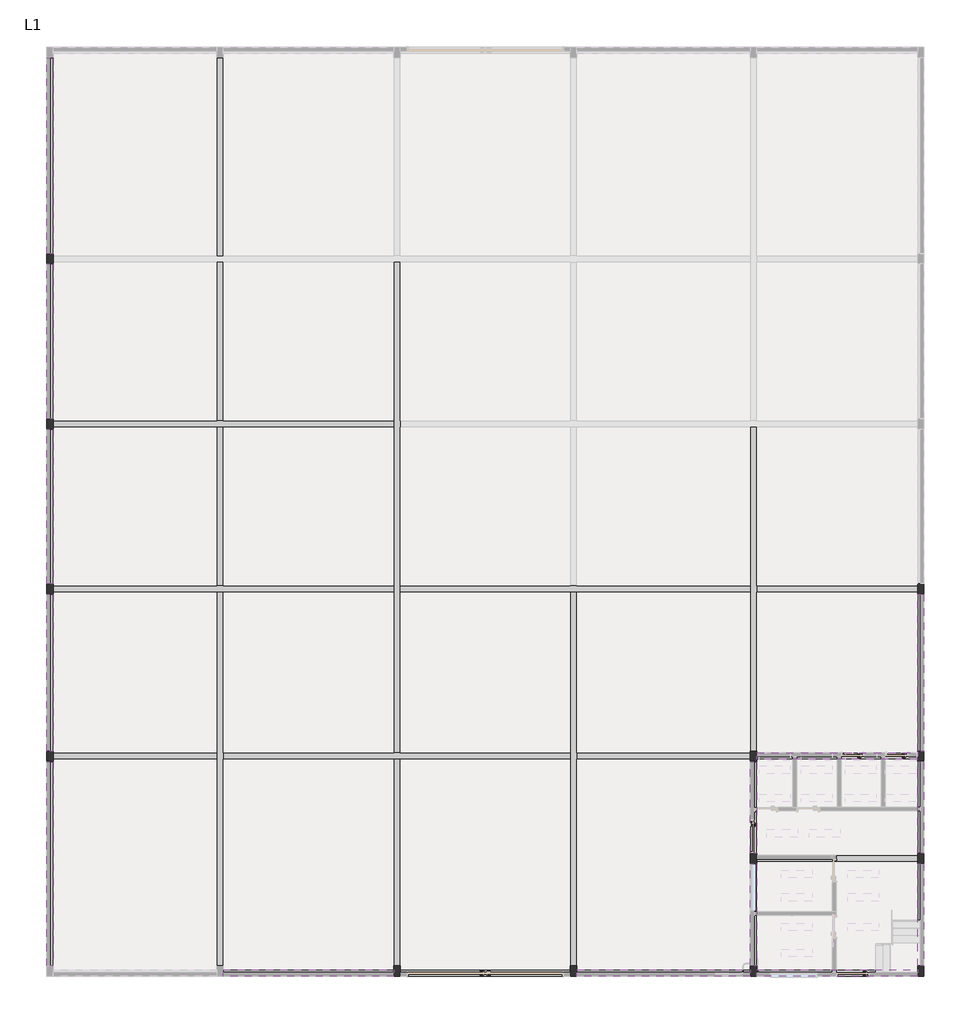
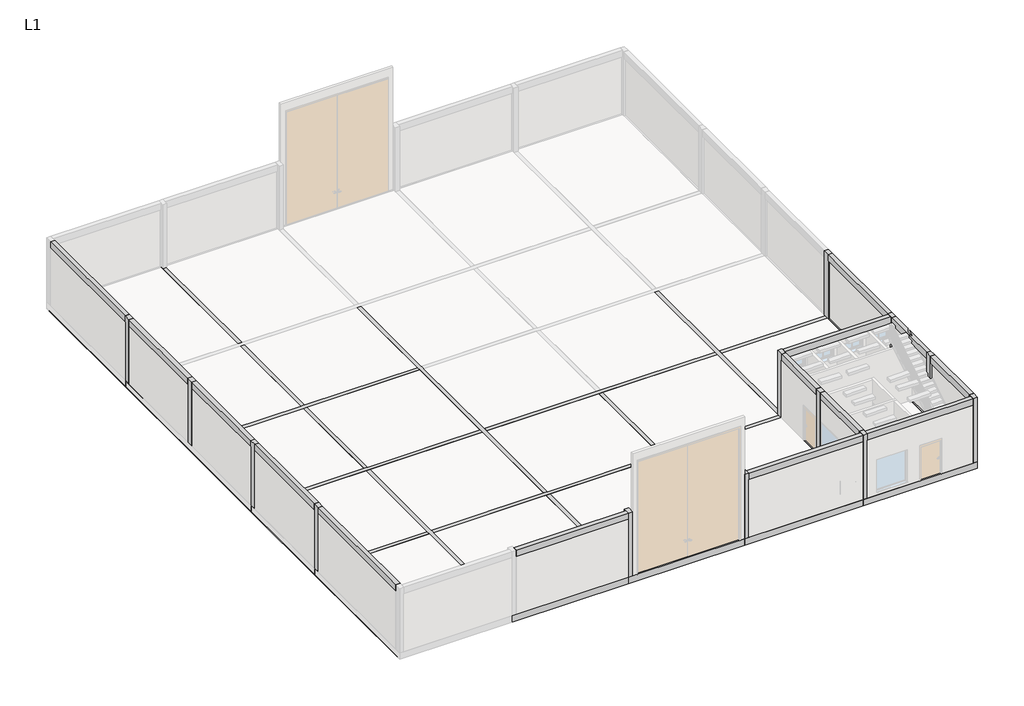
# One storey, part 2 of 4: 45 beams, 13 columns.
"""IFC4 building model written with IfcOpenShell, lengths in millimetres."""

from ifc_helpers import new_model, si_unit, frame, origin, place, context, project, spatial, polyline, outline, extrude, faceted_brep, element, save

model = new_model("IFC4")

# Units and contexts
model_context = context("Model", 3, world=origin())
ifc_project = project(units=[si_unit("LENGTHUNIT", "METRE", prefix="MILLI")], contexts=[model_context])

# Site, building, storey
site = spatial("IfcSite", under=ifc_project)
building = spatial("IfcBuilding", under=site)
storey = spatial("IfcBuildingStorey", under=building, Name="L1", Elevation=0.0)

# Beams
placement = place(None, origin())
element("IfcBeam", 1, ObjectType="M_Hormigón-Viga rectangular : 250 x 400mm", at=placement, inside=storey, context=model_context, shape_type="Brep", body=[
    faceted_brep([(17000.0, -3125.0, 0.0), (17000.0, -2875.0, 0.0), (16750.0, -2875.0, 0.0), (10525.0, -2875.0, 0.0), (10525.0, -3125.0, 0.0), (16750.0, -3125.0, 0.0), (17000.0, -2875.0, -400.0), (16750.0, -2875.0, -400.0), (10525.0, -2875.0, -400.0), (10525.0, -2875.0, -350.0), (17000.0, -3125.0, -400.0), (16750.0, -3125.0, -400.0), (10525.0, -3125.0, -400.0), (10525.0, -3125.0, -350.0)], [[[0, 1, 2, 3, 4, 5]], [[1, 6, 7, 8, 9, 3, 2]], [[6, 10, 11, 12, 8, 7]], [[10, 0, 5, 4, 13, 12, 11]], [[1, 0, 10, 6]], [[4, 3, 9, 8, 12, 13]]]),
])
element("IfcBeam", 2, ObjectType="M_Hormigón-Viga rectangular : 250 x 400mm", at=placement, inside=storey, context=model_context, shape_type="Brep", body=[
    faceted_brep([(10275.0, -9345.0, 0.0), (10275.0, -9595.0, 0.0), (10525.0, -9595.0, 0.0), (16750.0, -9595.0, 0.0), (17000.0, -9595.0, 0.0), (17000.0, -9345.0, 0.0), (16750.0, -9345.0, 0.0), (10525.0, -9345.0, 0.0), (10275.0, -9345.0, -400.0), (17000.0, -9345.0, -400.0), (16750.0, -9345.0, -400.0), (10525.0, -9345.0, -400.0), (10275.0, -9595.0, -400.0), (17000.0, -9595.0, -400.0), (16750.0, -9595.0, -400.0), (10525.0, -9595.0, -400.0)], [[[0, 1, 2, 3, 4, 5, 6, 7]], [[8, 0, 7, 6, 5, 9, 10, 11]], [[12, 8, 11, 10, 9, 13, 14, 15]], [[1, 12, 15, 14, 13, 4, 3, 2]], [[1, 0, 8, 12]], [[5, 4, 13, 9]]]),
])
element("IfcBeam", 3, ObjectType="M_Hormigón-Viga rectangular : 250 x 400mm", at=placement, inside=storey, context=model_context, shape_type="Brep", body=[
    faceted_brep([(10275.0, -9595.0, 0.0), (10275.0, -9345.0, 0.0), (3550.0, -9345.0, 0.0), (3550.0, -9595.0, 0.0), (10275.0, -9345.0, -350.0), (10275.0, -9345.0, -400.0), (3550.0, -9345.0, -400.0), (3550.0, -9345.0, -350.0), (10275.0, -9595.0, -400.0), (3550.0, -9595.0, -400.0), (10275.0, -9595.0, -350.0), (3550.0, -9595.0, -350.0)], [[[0, 1, 2, 3]], [[1, 4, 5, 6, 7, 2]], [[5, 8, 9, 6]], [[8, 10, 0, 3, 11, 9]], [[1, 0, 10, 8, 5, 4]], [[3, 2, 7, 6, 9, 11]]]),
])
element("IfcBeam", 4, ObjectType="M_Hormigón-Viga rectangular : 250 x 400mm", at=placement, inside=storey, context=model_context, shape_type="Brep", body=[
    faceted_brep([(10275.0, -17750.0, 0.0), (10275.0, -18000.0, 0.0), (17000.0, -18000.0, 0.0), (17000.0, -17750.0, 0.0), (16750.0, -17750.0, 0.0), (10525.0, -17750.0, 0.0), (10275.0, -17750.0, -400.0), (17000.0, -17750.0, -400.0), (16750.0, -17750.0, -400.0), (10525.0, -17750.0, -400.0), (10275.0, -18000.0, -400.0), (17000.0, -18000.0, -400.0)], [[[0, 1, 2, 3, 4, 5]], [[6, 0, 5, 4, 3, 7, 8, 9]], [[10, 6, 9, 8, 7, 11]], [[1, 10, 11, 2]], [[1, 0, 6, 10]], [[3, 2, 11, 7]]]),
])
element("IfcBeam", 5, ObjectType="M_Hormigón-Viga rectangular : 250 x 400mm", at=placement, inside=storey, context=model_context, shape_type="Brep", body=[
    faceted_brep([(3300.0, -17750.0, 0.0), (3300.0, -18000.0, 0.0), (10275.0, -18000.0, 0.0), (10275.0, -17750.0, 0.0), (3550.0, -17750.0, 0.0), (3300.0, -17750.0, -400.0), (10275.0, -17750.0, -350.0), (10275.0, -17750.0, -400.0), (3550.0, -17750.0, -400.0), (3300.0, -18000.0, -400.0), (10275.0, -18000.0, -400.0)], [[[0, 1, 2, 3, 4]], [[5, 0, 4, 3, 6, 7, 8]], [[9, 5, 8, 7, 10]], [[1, 9, 10, 2]], [[1, 0, 5, 9]], [[3, 2, 10, 7, 6]]]),
])
element("IfcBeam", 6, ObjectType="M_Hormigón-Viga rectangular : 250 x 400mm", at=placement, inside=storey, context=model_context, shape_type="Brep", body=[
    faceted_brep([(-3550.0, -17750.0, 0.0), (-3550.0, -18000.0, 0.0), (3300.0, -18000.0, 0.0), (3300.0, -17750.0, 0.0), (-3300.0, -17750.0, 0.0), (-3550.0, -17750.0, -400.0), (3300.0, -17750.0, -350.0), (3300.0, -17750.0, -400.0), (-3300.0, -17750.0, -400.0), (-3550.0, -18000.0, -400.0), (3300.0, -18000.0, -400.0)], [[[0, 1, 2, 3, 4]], [[5, 0, 4, 3, 6, 7, 8]], [[9, 5, 8, 7, 10]], [[1, 9, 10, 2]], [[1, 0, 5, 9]], [[3, 2, 10, 7, 6]]]),
])
element("IfcBeam", 7, ObjectType="M_Hormigón-Viga rectangular : 250 x 400mm", at=placement, inside=storey, context=model_context, shape_type="Brep", body=[
    faceted_brep([(-10400.0, -17750.0, 0.0), (-10400.0, -18000.0, 0.0), (-3550.0, -18000.0, 0.0), (-3550.0, -17750.0, 0.0), (-10150.0, -17750.0, 0.0), (-10400.0, -17750.0, -400.0), (-3550.0, -17750.0, -350.0), (-3550.0, -17750.0, -400.0), (-10150.0, -17750.0, -400.0), (-10400.0, -18000.0, -400.0), (-3550.0, -18000.0, -400.0)], [[[0, 1, 2, 3, 4]], [[5, 0, 4, 3, 6, 7, 8]], [[9, 5, 8, 7, 10]], [[1, 9, 10, 2]], [[3, 2, 10, 7, 6]], [[1, 0, 5, 9]]]),
])
element("IfcBeam", 8, ObjectType="M_Hormigón-Viga rectangular : 250 x 400mm", at=placement, inside=storey, context=model_context, shape_type="Brep", body=[
    faceted_brep([(-16750.0, -9345.0, 0.0), (-17000.0, -9345.0, 0.0), (-17000.0, -9685.0, 0.0), (-17000.0, -17600.0, 0.0), (-17000.0, -17750.0, 0.0), (-16750.0, -17750.0, 0.0), (-16750.0, -17600.0, 0.0), (-16750.0, -9685.0, 0.0), (-16750.0, -9595.0, 0.0), (-16750.0, -9345.0, -400.0), (-16750.0, -17750.0, -350.0), (-16750.0, -17750.0, -400.0), (-16750.0, -9595.0, -400.0), (-17000.0, -9345.0, -400.0), (-17000.0, -17750.0, -400.0)], [[[0, 1, 2, 3, 4, 5, 6, 7, 8]], [[9, 0, 8, 7, 6, 5, 10, 11, 12]], [[13, 9, 12, 11, 14]], [[1, 13, 14, 4, 3, 2]], [[1, 0, 9, 13]], [[5, 4, 14, 11, 10]]]),
])
element("IfcBeam", 9, ObjectType="M_Hormigón-Viga rectangular : 250 x 400mm", at=placement, inside=storey, context=model_context, shape_type="Brep", body=[
    faceted_brep([(-16750.0, -2875.0, 0.0), (-17000.0, -2875.0, 0.0), (-17000.0, -3200.0, 0.0), (-17000.0, -9285.0, 0.0), (-17000.0, -9345.0, 0.0), (-16750.0, -9345.0, 0.0), (-16750.0, -9285.0, 0.0), (-16750.0, -3200.0, 0.0), (-16750.0, -3125.0, 0.0), (-16750.0, -2875.0, -400.0), (-16750.0, -9345.0, -350.0), (-16750.0, -9345.0, -400.0), (-16750.0, -3125.0, -400.0), (-17000.0, -2875.0, -400.0), (-17000.0, -9345.0, -400.0)], [[[0, 1, 2, 3, 4, 5, 6, 7, 8]], [[9, 0, 8, 7, 6, 5, 10, 11, 12]], [[13, 9, 12, 11, 14]], [[1, 13, 14, 4, 3, 2]], [[1, 0, 9, 13]], [[5, 4, 14, 11, 10]]]),
])
element("IfcBeam", 10, ObjectType="M_Hormigón-Viga rectangular : 250 x 400mm", at=placement, inside=storey, context=model_context, shape_type="Brep", body=[
    faceted_brep([(-16750.0, 3525.0, 0.0), (-17000.0, 3525.0, 0.0), (-17000.0, 3200.0, 0.0), (-17000.0, -2800.0, 0.0), (-17000.0, -2875.0, 0.0), (-16750.0, -2875.0, 0.0), (-16750.0, -2800.0, 0.0), (-16750.0, 3200.0, 0.0), (-16750.0, 3275.0, 0.0), (-16750.0, 3525.0, -400.0), (-16750.0, -2875.0, -350.0), (-16750.0, -2875.0, -400.0), (-16750.0, 3275.0, -400.0), (-17000.0, 3525.0, -400.0), (-17000.0, -2875.0, -400.0)], [[[0, 1, 2, 3, 4, 5, 6, 7, 8]], [[9, 0, 8, 7, 6, 5, 10, 11, 12]], [[13, 9, 12, 11, 14]], [[1, 13, 14, 4, 3, 2]], [[1, 0, 9, 13]], [[5, 4, 14, 11, 10]]]),
])
element("IfcBeam", 11, ObjectType="M_Hormigón-Viga rectangular : 250 x 400mm", at=placement, inside=storey, context=model_context, shape_type="Brep", body=[
    faceted_brep([(-16750.0, 9925.0, 0.0), (-17000.0, 9925.0, 0.0), (-17000.0, 9600.0, 0.0), (-17000.0, 3600.0, 0.0), (-17000.0, 3525.0, 0.0), (-16750.0, 3525.0, 0.0), (-16750.0, 3600.0, 0.0), (-16750.0, 9600.0, 0.0), (-16750.0, 9675.0, 0.0), (-16750.0, 9925.0, -400.0), (-16750.0, 3525.0, -350.0), (-16750.0, 3525.0, -400.0), (-16750.0, 9675.0, -400.0), (-17000.0, 9925.0, -400.0), (-17000.0, 3525.0, -400.0)], [[[0, 1, 2, 3, 4, 5, 6, 7, 8]], [[9, 0, 8, 7, 6, 5, 10, 11, 12]], [[13, 9, 12, 11, 14]], [[1, 13, 14, 4, 3, 2]], [[1, 0, 9, 13]], [[5, 4, 14, 11, 10]]]),
])
element("IfcBeam", 12, ObjectType="M_Hormigón-Viga rectangular : 250 x 400mm", at=placement, inside=storey, context=model_context, shape_type="Brep", body=[
    faceted_brep([(-16750.0, 17750.0, 0.0), (-17000.0, 17750.0, 0.0), (-17000.0, 17600.0, 0.0), (-17000.0, 10000.0, 0.0), (-17000.0, 9925.0, 0.0), (-16750.0, 9925.0, 0.0), (-16750.0, 10000.0, 0.0), (-16750.0, 17600.0, 0.0), (-16750.0, 17750.0, -400.0), (-16750.0, 17750.0, -350.0), (-16750.0, 9925.0, -350.0), (-16750.0, 9925.0, -400.0), (-17000.0, 17750.0, -400.0), (-17000.0, 9925.0, -400.0)], [[[0, 1, 2, 3, 4, 5, 6, 7]], [[8, 9, 0, 7, 6, 5, 10, 11]], [[12, 8, 11, 13]], [[1, 12, 13, 4, 3, 2]], [[1, 0, 9, 8, 12]], [[5, 4, 13, 11, 10]]]),
])
element("IfcBeam", 13, ObjectType="M_Hormigón-Viga rectangular : 250 x 400mm", at=placement, inside=storey, context=model_context, shape_type="Brep", body=[
    faceted_brep([(-3550.0, -17750.0, 0.0), (-3300.0, -17750.0, 0.0), (-3300.0, -9595.0, 0.0), (-3550.0, -9595.0, 0.0), (-3300.0, -17750.0, -350.0), (-3300.0, -17750.0, -400.0), (-3300.0, -9595.0, -400.0), (-3300.0, -9595.0, -350.0), (-3550.0, -17750.0, -400.0), (-3550.0, -9595.0, -400.0), (-3550.0, -17750.0, -350.0), (-3550.0, -9595.0, -350.0)], [[[0, 1, 2, 3]], [[1, 4, 5, 6, 7, 2]], [[5, 8, 9, 6]], [[8, 10, 0, 3, 11, 9]], [[1, 0, 10, 8, 5, 4]], [[3, 2, 7, 6, 9, 11]]]),
])
element("IfcBeam", 14, ObjectType="M_Hormigón-Viga rectangular : 250 x 400mm", at=placement, inside=storey, context=model_context, shape_type="Brep", body=[
    faceted_brep([(3300.0, -17750.0, 0.0), (3550.0, -17750.0, 0.0), (3550.0, -9595.0, 0.0), (3550.0, -9345.0, 0.0), (3550.0, -3125.0, 0.0), (3300.0, -3125.0, 0.0), (3300.0, -9345.0, 0.0), (3300.0, -9595.0, 0.0), (3550.0, -17750.0, -350.0), (3550.0, -17750.0, -400.0), (3550.0, -9595.0, -400.0), (3550.0, -9345.0, -400.0), (3550.0, -3125.0, -400.0), (3550.0, -3125.0, -350.0), (3300.0, -17750.0, -400.0), (3300.0, -9595.0, -400.0), (3300.0, -9345.0, -400.0), (3300.0, -3125.0, -400.0), (3300.0, -17750.0, -350.0), (3300.0, -3125.0, -350.0)], [[[0, 1, 2, 3, 4, 5, 6, 7]], [[1, 8, 9, 10, 11, 12, 13, 4, 3, 2]], [[9, 14, 15, 16, 17, 12, 11, 10]], [[14, 18, 0, 7, 6, 5, 19, 17, 16, 15]], [[1, 0, 18, 14, 9, 8]], [[5, 4, 13, 12, 17, 19]]]),
])
element("IfcBeam", 15, ObjectType="M_Hormigón-Viga rectangular : 250 x 400mm", at=placement, inside=storey, context=model_context, shape_type="Brep", body=[
    faceted_brep([(10525.0, -13315.5675387, 0.0), (10275.0, -13315.5675387, 0.0), (10275.0, -17750.0, 0.0), (10525.0, -17750.0, 0.0), (10525.0, -13565.5675387, 0.0), (10525.0, -13315.5675387, -400.0), (10525.0, -17750.0, -350.0), (10525.0, -17750.0, -400.0), (10275.0, -13315.5675387, -400.0), (10275.0, -17750.0, -400.0), (10275.0, -17750.0, -350.0)], [[[0, 1, 2, 3, 4]], [[5, 0, 4, 3, 6, 7]], [[8, 5, 7, 9]], [[1, 8, 9, 10, 2]], [[3, 2, 10, 9, 7, 6]], [[1, 0, 5, 8]]]),
])
element("IfcBeam", 16, ObjectType="M_Hormigón-Viga rectangular : 250 x 400mm", at=placement, inside=storey, context=model_context, shape_type="Brep", body=[
    faceted_brep([(10525.0, -9595.0, 0.0), (10275.0, -9595.0, 0.0), (10275.0, -13315.5675387, 0.0), (10525.0, -13315.5675387, 0.0), (10525.0, -9595.0, -400.0), (10525.0, -9595.0, -350.0), (10525.0, -13315.5675387, -350.0), (10525.0, -13315.5675387, -400.0), (10275.0, -9595.0, -400.0), (10275.0, -13315.5675387, -400.0), (10275.0, -9595.0, -350.0)], [[[0, 1, 2, 3]], [[4, 5, 0, 3, 6, 7]], [[8, 4, 7, 9]], [[1, 10, 8, 9, 2]], [[1, 0, 5, 4, 8, 10]], [[3, 2, 9, 7, 6]]]),
])
element("IfcBeam", 17, ObjectType="M_Hormigón-Viga rectangular : 250 x 400mm", at=placement, inside=storey, context=model_context, shape_type="Brep", body=[
    faceted_brep([(10275.0, -9345.0, 0.0), (10525.0, -9345.0, 0.0), (10525.0, -3125.0, 0.0), (10525.0, -2875.0, 0.0), (10525.0, 3275.0, 0.0), (10275.0, 3275.0, 0.0), (10275.0, -2875.0, 0.0), (10275.0, -3125.0, 0.0), (10525.0, -9345.0, -350.0), (10525.0, -9345.0, -400.0), (10525.0, -3125.0, -400.0), (10525.0, -2875.0, -400.0), (10525.0, 3275.0, -400.0), (10525.0, 3275.0, -350.0), (10275.0, -9345.0, -400.0), (10275.0, -3125.0, -400.0), (10275.0, -2875.0, -400.0), (10275.0, 3275.0, -400.0), (10275.0, -9345.0, -350.0), (10275.0, 3275.0, -350.0)], [[[0, 1, 2, 3, 4, 5, 6, 7]], [[1, 8, 9, 10, 11, 12, 13, 4, 3, 2]], [[9, 14, 15, 16, 17, 12, 11, 10]], [[14, 18, 0, 7, 6, 5, 19, 17, 16, 15]], [[1, 0, 18, 14, 9, 8]], [[5, 4, 13, 12, 17, 19]]]),
])
element("IfcBeam", 18, ObjectType="M_Hormigón-Viga rectangular : 250 x 400mm", at=placement, inside=storey, context=model_context, shape_type="Brep", body=[
    faceted_brep([(17000.0, -13315.5675387, 0.0), (16750.0, -13315.5675387, 0.0), (16750.0, -13565.5675387, 0.0), (16750.0, -13640.5675387, 0.0), (16750.0, -17600.0, 0.0), (16750.0, -17750.0, 0.0), (17000.0, -17750.0, 0.0), (17000.0, -17600.0, 0.0), (17000.0, -13640.5675387, 0.0), (17000.0, -13315.5675387, -400.0), (17000.0, -17750.0, -400.0), (16750.0, -13315.5675387, -400.0), (16750.0, -17750.0, -400.0), (16750.0, -13565.5675387, -400.0), (16750.0, -17750.0, -350.0)], [[[0, 1, 2, 3, 4, 5, 6, 7, 8]], [[9, 0, 8, 7, 6, 10]], [[11, 9, 10, 12, 13]], [[1, 11, 13, 12, 14, 5, 4, 3, 2]], [[6, 5, 14, 12, 10]], [[1, 0, 9, 11]]]),
])
element("IfcBeam", 19, ObjectType="M_Hormigón-Viga rectangular : 250 x 400mm", at=placement, inside=storey, context=model_context, shape_type="Brep", body=[
    faceted_brep([(17000.0, -9595.0, 0.0), (16750.0, -9595.0, 0.0), (16750.0, -9685.0, 0.0), (16750.0, -13240.5675387, 0.0), (16750.0, -13315.5675387, 0.0), (17000.0, -13315.5675387, 0.0), (17000.0, -13240.5675387, 0.0), (17000.0, -9685.0, 0.0), (17000.0, -9595.0, -400.0), (17000.0, -13315.5675387, -400.0), (16750.0, -9595.0, -400.0), (16750.0, -13315.5675387, -400.0), (16750.0, -9595.0, -350.0), (16750.0, -13315.5675387, -350.0)], [[[0, 1, 2, 3, 4, 5, 6, 7]], [[8, 0, 7, 6, 5, 9]], [[10, 8, 9, 11]], [[1, 12, 10, 11, 13, 4, 3, 2]], [[1, 0, 8, 10, 12]], [[5, 4, 13, 11, 9]]]),
])
element("IfcBeam", 20, ObjectType="M_Hormigón-Viga rectangular : 250 x 400mm", at=placement, inside=storey, context=model_context, shape_type="Brep", body=[
    faceted_brep([(17000.0, -3125.0, 0.0), (16750.0, -3125.0, 0.0), (16750.0, -3200.0, 0.0), (16750.0, -9285.0, 0.0), (16750.0, -9345.0, 0.0), (17000.0, -9345.0, 0.0), (17000.0, -9285.0, 0.0), (17000.0, -3200.0, 0.0), (17000.0, -3125.0, -400.0), (17000.0, -9345.0, -400.0), (16750.0, -3125.0, -400.0), (16750.0, -9345.0, -400.0), (16750.0, -3125.0, -350.0), (16750.0, -9345.0, -350.0)], [[[0, 1, 2, 3, 4, 5, 6, 7]], [[8, 0, 7, 6, 5, 9]], [[10, 8, 9, 11]], [[1, 12, 10, 11, 13, 4, 3, 2]], [[1, 0, 8, 10, 12]], [[5, 4, 13, 11, 9]]]),
])
element("IfcBeam", 21, ObjectType="M_Hormigón-Viga rectangular : 250 x 400mm", at=placement, inside=storey, context=model_context, shape_type="Brep", body=[
    faceted_brep([(-10400.0, -17750.0, 0.0), (-10150.0, -17750.0, 0.0), (-10150.0, -9595.0, 0.0), (-10150.0, -9345.0, 0.0), (-10150.0, -3125.0, 0.0), (-10400.0, -3125.0, 0.0), (-10400.0, -9345.0, 0.0), (-10400.0, -9595.0, 0.0), (-10150.0, -17750.0, -350.0), (-10150.0, -17750.0, -400.0), (-10150.0, -9595.0, -400.0), (-10150.0, -9345.0, -400.0), (-10150.0, -3125.0, -400.0), (-10150.0, -3125.0, -350.0), (-10400.0, -17750.0, -400.0), (-10400.0, -9595.0, -400.0), (-10400.0, -9345.0, -400.0), (-10400.0, -3125.0, -400.0), (-10400.0, -17750.0, -350.0), (-10400.0, -3125.0, -350.0)], [[[0, 1, 2, 3, 4, 5, 6, 7]], [[1, 8, 9, 10, 11, 12, 13, 4, 3, 2]], [[9, 14, 15, 16, 17, 12, 11, 10]], [[14, 18, 0, 7, 6, 5, 19, 17, 16, 15]], [[1, 0, 18, 14, 9, 8]], [[5, 4, 13, 12, 17, 19]]]),
])
element("IfcBeam", 22, ObjectType="M_Hormigón-Viga rectangular : 250 x 400mm", at=placement, inside=storey, context=model_context, shape_type="Brep", body=[
    faceted_brep([(-16750.0, 3525.0, 0.0), (-16750.0, 3275.0, 0.0), (-10400.0, 3275.0, 0.0), (-10150.0, 3275.0, 0.0), (-3550.0, 3275.0, 0.0), (-3550.0, 3525.0, 0.0), (-10150.0, 3525.0, 0.0), (-10400.0, 3525.0, 0.0), (-16750.0, 3525.0, -400.0), (-16750.0, 3525.0, -350.0), (-3550.0, 3525.0, -350.0), (-3550.0, 3525.0, -400.0), (-10150.0, 3525.0, -400.0), (-10400.0, 3525.0, -400.0), (-16750.0, 3275.0, -400.0), (-3550.0, 3275.0, -400.0), (-10150.0, 3275.0, -400.0), (-10400.0, 3275.0, -400.0), (-16750.0, 3275.0, -350.0), (-3550.0, 3275.0, -350.0)], [[[0, 1, 2, 3, 4, 5, 6, 7]], [[8, 9, 0, 7, 6, 5, 10, 11, 12, 13]], [[14, 8, 13, 12, 11, 15, 16, 17]], [[1, 18, 14, 17, 16, 15, 19, 4, 3, 2]], [[1, 0, 9, 8, 14, 18]], [[5, 4, 19, 15, 11, 10]]]),
])
element("IfcBeam", 23, ObjectType="M_Hormigón-Viga rectangular : 250 x 400mm", at=placement, inside=storey, context=model_context, shape_type="Brep", body=[
    faceted_brep([(-16750.0, -2875.0, 0.0), (-16750.0, -3125.0, 0.0), (-10400.0, -3125.0, 0.0), (-10150.0, -3125.0, 0.0), (-3550.0, -3125.0, 0.0), (-3550.0, -2875.0, 0.0), (-10150.0, -2875.0, 0.0), (-10400.0, -2875.0, 0.0), (-16750.0, -2875.0, -400.0), (-16750.0, -2875.0, -350.0), (-3550.0, -2875.0, -350.0), (-3550.0, -2875.0, -400.0), (-10150.0, -2875.0, -400.0), (-10400.0, -2875.0, -400.0), (-16750.0, -3125.0, -400.0), (-3550.0, -3125.0, -400.0), (-10150.0, -3125.0, -400.0), (-10400.0, -3125.0, -400.0), (-16750.0, -3125.0, -350.0), (-3550.0, -3125.0, -350.0)], [[[0, 1, 2, 3, 4, 5, 6, 7]], [[8, 9, 0, 7, 6, 5, 10, 11, 12, 13]], [[14, 8, 13, 12, 11, 15, 16, 17]], [[1, 18, 14, 17, 16, 15, 19, 4, 3, 2]], [[1, 0, 9, 8, 14, 18]], [[5, 4, 19, 15, 11, 10]]]),
])
element("IfcBeam", 24, ObjectType="M_Hormigón-Viga rectangular : 250 x 400mm", at=placement, inside=storey, context=model_context, shape_type="Brep", body=[
    faceted_brep([(-3300.0, -2875.0, 0.0), (-3300.0, -3125.0, 0.0), (3300.0, -3125.0, 0.0), (3550.0, -3125.0, 0.0), (10275.0, -3125.0, 0.0), (10275.0, -2875.0, 0.0), (3550.0, -2875.0, 0.0), (3300.0, -2875.0, 0.0), (-3300.0, -2875.0, -400.0), (-3300.0, -2875.0, -350.0), (10275.0, -2875.0, -350.0), (10275.0, -2875.0, -400.0), (3550.0, -2875.0, -400.0), (3300.0, -2875.0, -400.0), (-3300.0, -3125.0, -400.0), (10275.0, -3125.0, -400.0), (3550.0, -3125.0, -400.0), (3300.0, -3125.0, -400.0), (-3300.0, -3125.0, -350.0), (10275.0, -3125.0, -350.0)], [[[0, 1, 2, 3, 4, 5, 6, 7]], [[8, 9, 0, 7, 6, 5, 10, 11, 12, 13]], [[14, 8, 13, 12, 11, 15, 16, 17]], [[1, 18, 14, 17, 16, 15, 19, 4, 3, 2]], [[1, 0, 9, 8, 14, 18]], [[5, 4, 19, 15, 11, 10]]]),
])
element("IfcBeam", 25, ObjectType="M_Hormigón-Viga rectangular : 250 x 400mm", at=placement, inside=storey, context=model_context, shape_type="Brep", body=[
    faceted_brep([(-3300.0, 9675.0, 0.0), (-3550.0, 9675.0, 0.0), (-3550.0, 3525.0, 0.0), (-3550.0, 3275.0, 0.0), (-3550.0, -2875.0, 0.0), (-3550.0, -3125.0, 0.0), (-3550.0, -9345.0, 0.0), (-3300.0, -9345.0, 0.0), (-3300.0, -3125.0, 0.0), (-3300.0, -2875.0, 0.0), (-3300.0, 3275.0, 0.0), (-3300.0, 3525.0, 0.0), (-3300.0, 9675.0, -400.0), (-3300.0, 9675.0, -350.0), (-3300.0, -9345.0, -350.0), (-3300.0, -9345.0, -400.0), (-3300.0, -3125.0, -400.0), (-3300.0, -2875.0, -400.0), (-3300.0, 3275.0, -400.0), (-3300.0, 3525.0, -400.0), (-3550.0, 9675.0, -400.0), (-3550.0, -9345.0, -400.0), (-3550.0, -3125.0, -400.0), (-3550.0, -2875.0, -400.0), (-3550.0, 3275.0, -400.0), (-3550.0, 3525.0, -400.0), (-3550.0, 9675.0, -350.0), (-3550.0, -9345.0, -350.0)], [[[0, 1, 2, 3, 4, 5, 6, 7, 8, 9, 10, 11]], [[12, 13, 0, 11, 10, 9, 8, 7, 14, 15, 16, 17, 18, 19]], [[20, 12, 19, 18, 17, 16, 15, 21, 22, 23, 24, 25]], [[1, 26, 20, 25, 24, 23, 22, 21, 27, 6, 5, 4, 3, 2]], [[1, 0, 13, 12, 20, 26]], [[7, 6, 27, 21, 15, 14]]]),
])
element("IfcBeam", 26, ObjectType="M_Hormigón-Viga rectangular : 250 x 400mm", at=placement, inside=storey, context=model_context, shape_type="Brep", body=[
    faceted_brep([(3300.0, -9595.0, 0.0), (3300.0, -9345.0, 0.0), (-3300.0, -9345.0, 0.0), (-3550.0, -9345.0, 0.0), (-10150.0, -9345.0, 0.0), (-10150.0, -9595.0, 0.0), (-3550.0, -9595.0, 0.0), (-3300.0, -9595.0, 0.0), (3300.0, -9345.0, -350.0), (3300.0, -9345.0, -400.0), (-3300.0, -9345.0, -400.0), (-3550.0, -9345.0, -400.0), (-10150.0, -9345.0, -400.0), (-10150.0, -9345.0, -350.0), (3300.0, -9595.0, -400.0), (-3300.0, -9595.0, -400.0), (-3550.0, -9595.0, -400.0), (-10150.0, -9595.0, -400.0), (3300.0, -9595.0, -350.0), (-10150.0, -9595.0, -350.0)], [[[0, 1, 2, 3, 4, 5, 6, 7]], [[1, 8, 9, 10, 11, 12, 13, 4, 3, 2]], [[9, 14, 15, 16, 17, 12, 11, 10]], [[14, 18, 0, 7, 6, 5, 19, 17, 16, 15]], [[1, 0, 18, 14, 9, 8]], [[5, 4, 13, 12, 17, 19]]]),
])
element("IfcBeam", 27, ObjectType="M_Hormigón-Viga rectangular : 250 x 400mm", at=placement, inside=storey, context=model_context, shape_type="Brep", body=[
    faceted_brep([(-10150.0, 17750.0, 0.0), (-10400.0, 17750.0, 0.0), (-10400.0, 9925.0, 0.0), (-10150.0, 9925.0, 0.0), (-10150.0, 17750.0, -400.0), (-10150.0, 17750.0, -350.0), (-10150.0, 9925.0, -350.0), (-10150.0, 9925.0, -400.0), (-10400.0, 17750.0, -400.0), (-10400.0, 9925.0, -400.0), (-10400.0, 17750.0, -350.0), (-10400.0, 9925.0, -350.0)], [[[0, 1, 2, 3]], [[4, 5, 0, 3, 6, 7]], [[8, 4, 7, 9]], [[1, 10, 8, 9, 11, 2]], [[1, 0, 5, 4, 8, 10]], [[3, 2, 11, 9, 7, 6]]]),
])
element("IfcBeam", 28, ObjectType="M_Hormigón-Viga rectangular : 250 x 400mm", at=placement, inside=storey, context=model_context, shape_type="Brep", body=[
    faceted_brep([(-10150.0, 9675.0, 0.0), (-10400.0, 9675.0, 0.0), (-10400.0, 3525.0, 0.0), (-10150.0, 3525.0, 0.0), (-10150.0, 9675.0, -400.0), (-10150.0, 9675.0, -350.0), (-10150.0, 3525.0, -350.0), (-10150.0, 3525.0, -400.0), (-10400.0, 9675.0, -400.0), (-10400.0, 3525.0, -400.0), (-10400.0, 9675.0, -350.0), (-10400.0, 3525.0, -350.0)], [[[0, 1, 2, 3]], [[4, 5, 0, 3, 6, 7]], [[8, 4, 7, 9]], [[1, 10, 8, 9, 11, 2]], [[1, 0, 5, 4, 8, 10]], [[3, 2, 11, 9, 7, 6]]]),
])
element("IfcBeam", 29, ObjectType="M_Hormigón-Viga rectangular : 250 x 400mm", at=placement, inside=storey, context=model_context, shape_type="Brep", body=[
    faceted_brep([(-10150.0, 3275.0, 0.0), (-10400.0, 3275.0, 0.0), (-10400.0, -2875.0, 0.0), (-10150.0, -2875.0, 0.0), (-10150.0, 3275.0, -400.0), (-10150.0, 3275.0, -350.0), (-10150.0, -2875.0, -350.0), (-10150.0, -2875.0, -400.0), (-10400.0, 3275.0, -400.0), (-10400.0, -2875.0, -400.0), (-10400.0, 3275.0, -350.0), (-10400.0, -2875.0, -350.0)], [[[0, 1, 2, 3]], [[4, 5, 0, 3, 6, 7]], [[8, 4, 7, 9]], [[1, 10, 8, 9, 11, 2]], [[1, 0, 5, 4, 8, 10]], [[3, 2, 11, 9, 7, 6]]]),
])
element("IfcBeam", 30, ObjectType="M_Hormigón-Viga rectangular : 250 x 400mm", at=placement, inside=storey, context=model_context, shape_type="Brep", body=[
    faceted_brep([(-16750.0, -9345.0, 0.0), (-16750.0, -9595.0, 0.0), (-10400.0, -9595.0, 0.0), (-10400.0, -9345.0, 0.0), (-16750.0, -9345.0, -400.0), (-16750.0, -9345.0, -350.0), (-10400.0, -9345.0, -350.0), (-10400.0, -9345.0, -400.0), (-16750.0, -9595.0, -400.0), (-10400.0, -9595.0, -400.0), (-16750.0, -9595.0, -350.0), (-10400.0, -9595.0, -350.0)], [[[0, 1, 2, 3]], [[4, 5, 0, 3, 6, 7]], [[8, 4, 7, 9]], [[1, 10, 8, 9, 11, 2]], [[1, 0, 5, 4, 8, 10]], [[3, 2, 11, 9, 7, 6]]]),
])
element("IfcBeam", 31, ObjectType="M_Hormigón-Viga rectangular : 250 x 400mm", at=placement, inside=storey, context=model_context, shape_type="Brep", body=[
    faceted_brep([(10525.0, -13315.5675387, 0.0), (10525.0, -13565.5675387, 0.0), (16750.0, -13565.5675387, 0.0), (16750.0, -13315.5675387, 0.0), (10525.0, -13565.5675387, -350.0), (10525.0, -13565.5675387, -400.0), (16750.0, -13565.5675387, -400.0), (16750.0, -13565.5675387, -350.0), (10525.0, -13315.5675387, -400.0), (16750.0, -13315.5675387, -400.0), (10525.0, -13315.5675387, -350.0), (16750.0, -13315.5675387, -350.0)], [[[0, 1, 2, 3]], [[1, 4, 5, 6, 7, 2]], [[5, 8, 9, 6]], [[8, 10, 0, 3, 11, 9]], [[1, 0, 10, 8, 5, 4]], [[3, 2, 7, 6, 9, 11]]]),
])
element("IfcBeam", 32, ObjectType="M_Hormigón-Viga rectangular : 250 x 400mm", at=placement, inside=storey, context=model_context, shape_type="Brep", body=[
    faceted_brep([(10525.0, -9345.0, 4000.0), (10525.0, -9595.0, 4000.0), (16750.0, -9595.0, 4000.0), (16750.0, -9345.0, 4000.0), (10525.0, -9345.0, 3600.0), (10525.0, -9345.0, 3800.0), (16750.0, -9345.0, 3800.0), (16750.0, -9345.0, 3600.0), (10525.0, -9595.0, 3600.0), (16750.0, -9595.0, 3600.0), (10525.0, -9595.0, 3800.0), (16750.0, -9595.0, 3800.0)], [[[0, 1, 2, 3]], [[4, 5, 0, 3, 6, 7]], [[8, 4, 7, 9]], [[1, 10, 8, 9, 11, 2]], [[1, 0, 5, 4, 8, 10]], [[3, 2, 11, 9, 7, 6]]]),
])
element("IfcBeam", 33, ObjectType="M_Hormigón-Viga rectangular : 250 x 400mm", at=placement, inside=storey, context=model_context, shape_type="Brep", body=[
    faceted_brep([(10525.0, -17750.0, 4000.0), (10525.0, -18000.0, 4000.0), (16750.0, -18000.0, 4000.0), (16750.0, -17750.0, 4000.0), (15647.5726879, -17750.0, 4000.0), (10525.0, -17750.0, 3600.0), (10525.0, -17750.0, 3800.0), (16750.0, -17750.0, 3600.0), (10525.0, -18000.0, 3600.0), (16750.0, -18000.0, 3600.0)], [[[0, 1, 2, 3, 4]], [[5, 6, 0, 4, 3, 7]], [[8, 5, 7, 9]], [[1, 8, 9, 2]], [[1, 0, 6, 5, 8]], [[3, 2, 9, 7]]]),
])
element("IfcBeam", 34, ObjectType="M_Hormigón-Viga rectangular : 250 x 400mm", at=placement, inside=storey, context=model_context, shape_type="SweptSolid", body=[
    extrude(outline(polyline([(3550.0, -18000.0), (3550.0, -17750.0), (10275.0, -17750.0), (10275.0, -18000.0), (3550.0, -18000.0)])), frame((0.0, 0.0, 3600.0), z_axis=(0.0, 0.0, 1.0), x_axis=(1.0, 0.0, 0.0)), (0.0, 0.0, 1.0), 400.0),
])
element("IfcBeam", 35, ObjectType="M_Hormigón-Viga rectangular : 250 x 400mm", at=placement, inside=storey, context=model_context, shape_type="SweptSolid", body=[
    extrude(outline(polyline([(-3550.0, -17750.0), (-3550.0, -18000.0), (-10150.0, -18000.0), (-10150.0, -17750.0), (-3550.0, -17750.0)])), frame((0.0, 0.0, 3600.0), z_axis=(0.0, 0.0, 1.0), x_axis=(1.0, 0.0, 0.0)), (0.0, 0.0, 1.0), 400.0),
])
element("IfcBeam", 36, ObjectType="M_Hormigón-Viga rectangular : 250 x 400mm", at=placement, inside=storey, context=model_context, shape_type="SweptSolid", body=[
    extrude(outline(polyline([(-17000.0, -9685.0), (-16750.0, -9685.0), (-16750.0, -17600.0), (-17000.0, -17600.0), (-17000.0, -9685.0)])), frame((0.0, 0.0, 3600.0), z_axis=(0.0, 0.0, 1.0), x_axis=(1.0, 0.0, 0.0)), (0.0, 0.0, 1.0), 400.0),
])
element("IfcBeam", 37, ObjectType="M_Hormigón-Viga rectangular : 250 x 400mm", at=placement, inside=storey, context=model_context, shape_type="SweptSolid", body=[
    extrude(outline(polyline([(-17000.0, -3200.0), (-16750.0, -3200.0), (-16750.0, -9285.0), (-17000.0, -9285.0), (-17000.0, -3200.0)])), frame((0.0, 0.0, 3600.0), z_axis=(0.0, 0.0, 1.0), x_axis=(1.0, 0.0, 0.0)), (0.0, 0.0, 1.0), 400.0),
])
element("IfcBeam", 38, ObjectType="M_Hormigón-Viga rectangular : 250 x 400mm", at=placement, inside=storey, context=model_context, shape_type="SweptSolid", body=[
    extrude(outline(polyline([(-17000.0, 3200.0), (-16750.0, 3200.0), (-16750.0, -2800.0), (-17000.0, -2800.0), (-17000.0, 3200.0)])), frame((0.0, 0.0, 3600.0), z_axis=(0.0, 0.0, 1.0), x_axis=(1.0, 0.0, 0.0)), (0.0, 0.0, 1.0), 400.0),
])
element("IfcBeam", 39, ObjectType="M_Hormigón-Viga rectangular : 250 x 400mm", at=placement, inside=storey, context=model_context, shape_type="SweptSolid", body=[
    extrude(outline(polyline([(-17000.0, 9600.0), (-16750.0, 9600.0), (-16750.0, 3600.0), (-17000.0, 3600.0), (-17000.0, 9600.0)])), frame((0.0, 0.0, 3600.0), z_axis=(0.0, 0.0, 1.0), x_axis=(1.0, 0.0, 0.0)), (0.0, 0.0, 1.0), 400.0),
])
element("IfcBeam", 40, ObjectType="M_Hormigón-Viga rectangular : 250 x 400mm", at=placement, inside=storey, context=model_context, shape_type="SweptSolid", body=[
    extrude(outline(polyline([(-17000.0, 17600.0), (-16750.0, 17600.0), (-16750.0, 10000.0), (-17000.0, 10000.0), (-17000.0, 17600.0)])), frame((0.0, 0.0, 3600.0), z_axis=(0.0, 0.0, 1.0), x_axis=(1.0, 0.0, 0.0)), (0.0, 0.0, 1.0), 400.0),
])
element("IfcBeam", 41, ObjectType="M_Hormigón-Viga rectangular : 250 x 400mm", at=placement, inside=storey, context=model_context, shape_type="SweptSolid", body=[
    extrude(outline(polyline([(10525.0, -17600.0), (10275.0, -17600.0), (10275.0, -13640.5675387), (10525.0, -13640.5675387), (10525.0, -17600.0)])), frame((0.0, 0.0, 3600.0), z_axis=(0.0, 0.0, 1.0), x_axis=(1.0, 0.0, 0.0)), (0.0, 0.0, 1.0), 400.0),
])
element("IfcBeam", 42, ObjectType="M_Hormigón-Viga rectangular : 250 x 400mm", at=placement, inside=storey, context=model_context, shape_type="SweptSolid", body=[
    extrude(outline(polyline([(10275.0, -9685.0), (10525.0, -9685.0), (10525.0, -13240.5675387), (10275.0, -13240.5675387), (10275.0, -9685.0)])), frame((0.0, 0.0, 3600.0), z_axis=(0.0, 0.0, 1.0), x_axis=(1.0, 0.0, 0.0)), (0.0, 0.0, 1.0), 400.0),
])
element("IfcBeam", 43, ObjectType="M_Hormigón-Viga rectangular : 250 x 400mm", at=placement, inside=storey, context=model_context, shape_type="SweptSolid", body=[
    extrude(outline(polyline([(17000.0, -17600.0), (16750.0, -17600.0), (16750.0, -13640.5675387), (17000.0, -13640.5675387), (17000.0, -17600.0)])), frame((0.0, 0.0, 3600.0), z_axis=(0.0, 0.0, 1.0), x_axis=(1.0, 0.0, 0.0)), (0.0, 0.0, 1.0), 400.0),
])
element("IfcBeam", 44, ObjectType="M_Hormigón-Viga rectangular : 250 x 400mm", at=placement, inside=storey, context=model_context, shape_type="Brep", body=[
    faceted_brep([(17000.0, -9685.0, 4000.0), (16750.0, -9685.0, 4000.0), (16750.0, -11597.1858803, 4000.0), (16750.0, -13240.5675387, 4000.0), (17000.0, -13240.5675387, 4000.0), (17000.0, -9685.0, 3600.0), (17000.0, -13240.5675387, 3600.0), (16750.0, -9685.0, 3600.0), (16750.0, -13240.5675387, 3600.0)], [[[0, 1, 2, 3, 4]], [[5, 0, 4, 6]], [[7, 5, 6, 8]], [[1, 7, 8, 3, 2]], [[1, 0, 5, 7]], [[4, 3, 8, 6]]]),
])
element("IfcBeam", 45, ObjectType="M_Hormigón-Viga rectangular : 250 x 400mm", at=placement, inside=storey, context=model_context, shape_type="SweptSolid", body=[
    extrude(outline(polyline([(-3200.0, 4000.0), (-3200.0, 3600.0), (-9285.0, 3600.0), (-9285.0, 3800.0), (-9270.0, 3800.0), (-9270.0, 4000.0), (-3200.0, 4000.0)])), frame((16750.0, 0.0, 0.0), z_axis=(1.0, 0.0, 0.0), x_axis=(0.0, 1.0, 0.0)), (0.0, 0.0, 1.0), 250.0),
])

# Columns
element("IfcColumn", 46, ObjectType="M_Hormigón-Rectangular-Pilar : 250 x 400mm", at=placement, inside=storey, context=model_context, shape_type="Brep", body=[
    faceted_brep([(-17000.0, 9600.0, 0.0), (-17000.0, 9925.0, 0.0), (-17000.0, 10000.0, 0.0), (-16750.0, 10000.0, 0.0), (-16750.0, 9925.0, 0.0), (-16750.0, 9600.0, 0.0), (-17000.0, 9600.0, 4000.0), (-17000.0, 10000.0, 4000.0), (-16750.0, 10000.0, 4000.0), (-16750.0, 9600.0, 4000.0)], [[[0, 1, 2, 3, 4, 5]], [[6, 7, 2, 1, 0]], [[7, 8, 3, 2]], [[8, 9, 5, 4, 3]], [[9, 6, 0, 5]], [[6, 9, 8, 7]]]),
])
element("IfcColumn", 47, ObjectType="M_Hormigón-Rectangular-Pilar : 250 x 400mm", at=placement, inside=storey, context=model_context, shape_type="Brep", body=[
    faceted_brep([(-17000.0, 3200.0, 0.0), (-17000.0, 3525.0, 0.0), (-17000.0, 3600.0, 0.0), (-16750.0, 3600.0, 0.0), (-16750.0, 3525.0, 0.0), (-16750.0, 3200.0, 0.0), (-17000.0, 3200.0, 4000.0), (-17000.0, 3600.0, 4000.0), (-16750.0, 3600.0, 4000.0), (-16750.0, 3200.0, 4000.0)], [[[0, 1, 2, 3, 4, 5]], [[6, 7, 2, 1, 0]], [[7, 8, 3, 2]], [[8, 9, 5, 4, 3]], [[9, 6, 0, 5]], [[6, 9, 8, 7]]]),
])
element("IfcColumn", 48, ObjectType="M_Hormigón-Rectangular-Pilar : 250 x 400mm", at=placement, inside=storey, context=model_context, shape_type="Brep", body=[
    faceted_brep([(-17000.0, -3200.0, 0.0), (-17000.0, -2875.0, 0.0), (-17000.0, -2800.0, 0.0), (-16750.0, -2800.0, 0.0), (-16750.0, -2875.0, 0.0), (-16750.0, -3200.0, 0.0), (-17000.0, -3200.0, 4000.0), (-17000.0, -2800.0, 4000.0), (-16750.0, -2800.0, 4000.0), (-16750.0, -3200.0, 4000.0)], [[[0, 1, 2, 3, 4, 5]], [[6, 7, 2, 1, 0]], [[7, 8, 3, 2]], [[8, 9, 5, 4, 3]], [[9, 6, 0, 5]], [[6, 9, 8, 7]]]),
])
element("IfcColumn", 49, ObjectType="M_Hormigón-Rectangular-Pilar : 250 x 400mm", at=placement, inside=storey, context=model_context, shape_type="Brep", body=[
    faceted_brep([(16750.0, -3200.0, 0.0), (16750.0, -3125.0, 0.0), (16750.0, -2875.0, 0.0), (16750.0, -2800.0, 0.0), (17000.0, -2800.0, 0.0), (17000.0, -2875.0, 0.0), (17000.0, -3125.0, 0.0), (17000.0, -3200.0, 0.0), (16750.0, -3200.0, 4000.0), (16750.0, -2800.0, 4000.0), (17000.0, -2800.0, 4000.0), (17000.0, -3200.0, 4000.0)], [[[0, 1, 2, 3, 4, 5, 6, 7]], [[8, 9, 3, 2, 1, 0]], [[9, 10, 4, 3]], [[10, 11, 7, 6, 5, 4]], [[11, 8, 0, 7]], [[8, 11, 10, 9]]]),
])
element("IfcColumn", 50, ObjectType="M_Hormigón-Rectangular-Pilar : 250 x 400mm", at=placement, inside=storey, context=model_context, shape_type="Brep", body=[
    faceted_brep([(-17000.0, -9685.0, 0.0), (-17000.0, -9345.0, 0.0), (-17000.0, -9285.0, 0.0), (-16750.0, -9285.0, 0.0), (-16750.0, -9345.0, 0.0), (-16750.0, -9685.0, 0.0), (-17000.0, -9685.0, 4000.0), (-17000.0, -9285.0, 4000.0), (-16750.0, -9285.0, 4000.0), (-16750.0, -9685.0, 4000.0)], [[[0, 1, 2, 3, 4, 5]], [[6, 7, 2, 1, 0]], [[7, 8, 3, 2]], [[8, 9, 5, 4, 3]], [[9, 6, 0, 5]], [[6, 9, 8, 7]]]),
])
element("IfcColumn", 51, ObjectType="M_Hormigón-Rectangular-Pilar : 250 x 400mm", at=placement, inside=storey, context=model_context, shape_type="Brep", body=[
    faceted_brep([(10275.0, -9685.0, 0.0), (10275.0, -9595.0, 0.0), (10275.0, -9345.0, 0.0), (10275.0, -9285.0, 0.0), (10525.0, -9285.0, 0.0), (10525.0, -9345.0, 0.0), (10525.0, -9595.0, 0.0), (10525.0, -9685.0, 0.0), (10275.0, -9685.0, 4000.0), (10275.0, -9285.0, 4000.0), (10275.0, -9285.0, 3800.0), (10525.0, -9285.0, 4000.0), (10525.0, -9285.0, 3800.0), (10525.0, -9345.0, 4000.0), (10525.0, -9595.0, 4000.0), (10525.0, -9685.0, 4000.0)], [[[0, 1, 2, 3, 4, 5, 6, 7]], [[8, 9, 10, 3, 2, 1, 0]], [[9, 11, 12, 4, 3, 10]], [[11, 13, 14, 15, 7, 6, 5, 4, 12]], [[15, 8, 0, 7]], [[8, 15, 14, 13, 11, 9]]]),
])
element("IfcColumn", 52, ObjectType="M_Hormigón-Rectangular-Pilar : 250 x 400mm", at=placement, inside=storey, context=model_context, shape_type="Brep", body=[
    faceted_brep([(16750.0, -9685.0, 0.0), (16750.0, -9595.0, 0.0), (16750.0, -9345.0, 0.0), (16750.0, -9285.0, 0.0), (17000.0, -9285.0, 0.0), (17000.0, -9345.0, 0.0), (17000.0, -9595.0, 0.0), (17000.0, -9685.0, 0.0), (16750.0, -9685.0, 4000.0), (16750.0, -9595.0, 4000.0), (16750.0, -9345.0, 4000.0), (16750.0, -9285.0, 4000.0), (16750.0, -9285.0, 3800.0), (17000.0, -9285.0, 4000.0), (17000.0, -9285.0, 3800.0), (17000.0, -9685.0, 4000.0)], [[[0, 1, 2, 3, 4, 5, 6, 7]], [[8, 9, 10, 11, 12, 3, 2, 1, 0]], [[11, 13, 14, 4, 3, 12]], [[13, 15, 7, 6, 5, 4, 14]], [[15, 8, 0, 7]], [[8, 15, 13, 11, 10, 9]]]),
])
element("IfcColumn", 53, ObjectType="M_Hormigón-Rectangular-Pilar : 250 x 400mm", at=placement, inside=storey, context=model_context, shape_type="Brep", body=[
    faceted_brep([(-3550.0, -18000.0, 0.0), (-3550.0, -17750.0, 0.0), (-3550.0, -17600.0, 0.0), (-3300.0, -17600.0, 0.0), (-3300.0, -17750.0, 0.0), (-3300.0, -18000.0, 0.0), (-3550.0, -18000.0, 4000.0), (-3550.0, -17600.0, 4000.0), (-3300.0, -17600.0, 4000.0), (-3300.0, -18000.0, 4000.0)], [[[0, 1, 2, 3, 4, 5]], [[6, 7, 2, 1, 0]], [[7, 8, 3, 2]], [[8, 9, 5, 4, 3]], [[9, 6, 0, 5]], [[6, 9, 8, 7]]]),
])
element("IfcColumn", 54, ObjectType="M_Hormigón-Rectangular-Pilar : 250 x 400mm", at=placement, inside=storey, context=model_context, shape_type="Brep", body=[
    faceted_brep([(3300.0, -18000.0, 0.0), (3300.0, -17750.0, 0.0), (3300.0, -17600.0, 0.0), (3550.0, -17600.0, 0.0), (3550.0, -17750.0, 0.0), (3550.0, -18000.0, 0.0), (3300.0, -18000.0, 4000.0), (3300.0, -17600.0, 4000.0), (3550.0, -17600.0, 4000.0), (3550.0, -18000.0, 4000.0)], [[[0, 1, 2, 3, 4, 5]], [[6, 7, 2, 1, 0]], [[7, 8, 3, 2]], [[8, 9, 5, 4, 3]], [[9, 6, 0, 5]], [[6, 9, 8, 7]]]),
])
element("IfcColumn", 55, ObjectType="M_Hormigón-Rectangular-Pilar : 250 x 400mm", at=placement, inside=storey, context=model_context, shape_type="Brep", body=[
    faceted_brep([(10275.0, -18000.0, 0.0), (10275.0, -17750.0, 0.0), (10275.0, -17600.0, 0.0), (10525.0, -17600.0, 0.0), (10525.0, -17750.0, 0.0), (10525.0, -18000.0, 0.0), (10275.0, -18000.0, 4000.0), (10275.0, -17600.0, 4000.0), (10525.0, -17600.0, 4000.0), (10525.0, -17750.0, 4000.0), (10525.0, -18000.0, 4000.0)], [[[0, 1, 2, 3, 4, 5]], [[6, 7, 2, 1, 0]], [[7, 8, 3, 2]], [[8, 9, 10, 5, 4, 3]], [[10, 6, 0, 5]], [[6, 10, 9, 8, 7]]]),
])
element("IfcColumn", 56, ObjectType="M_Hormigón-Rectangular-Pilar : 250 x 400mm", at=placement, inside=storey, context=model_context, shape_type="Brep", body=[
    faceted_brep([(16750.0, -18000.0, 0.0), (16750.0, -17750.0, 0.0), (16750.0, -17600.0, 0.0), (17000.0, -17600.0, 0.0), (17000.0, -17750.0, 0.0), (17000.0, -18000.0, 0.0), (16750.0, -18000.0, 4000.0), (16750.0, -17600.0, 4000.0), (17000.0, -17600.0, 4000.0), (17000.0, -18000.0, 4000.0)], [[[0, 1, 2, 3, 4, 5]], [[6, 7, 2, 1, 0]], [[7, 8, 3, 2]], [[8, 9, 5, 4, 3]], [[9, 6, 0, 5]], [[6, 9, 8, 7]]]),
])
element("IfcColumn", 57, ObjectType="M_Hormigón-Rectangular-Pilar : 250 x 400mm", at=placement, inside=storey, context=model_context, shape_type="Brep", body=[
    faceted_brep([(10525.0, -13240.5675387, 0.0), (10525.0, -13315.5675387, 0.0), (10525.0, -13640.5675387, 0.0), (10275.0, -13640.5675387, 0.0), (10275.0, -13315.5675387, 0.0), (10275.0, -13240.5675387, 0.0), (10525.0, -13240.5675387, 4000.0), (10525.0, -13640.5675387, 4000.0), (10275.0, -13640.5675387, 4000.0), (10275.0, -13240.5675387, 4000.0)], [[[0, 1, 2, 3, 4, 5]], [[6, 7, 2, 1, 0]], [[7, 8, 3, 2]], [[8, 9, 5, 4, 3]], [[9, 6, 0, 5]], [[6, 9, 8, 7]]]),
])
element("IfcColumn", 58, ObjectType="M_Hormigón-Rectangular-Pilar : 250 x 400mm", at=placement, inside=storey, context=model_context, shape_type="Brep", body=[
    faceted_brep([(17000.0, -13240.5675387, 0.0), (17000.0, -13315.5675387, 0.0), (17000.0, -13640.5675387, 0.0), (16750.0, -13640.5675387, 0.0), (16750.0, -13315.5675387, 0.0), (16750.0, -13240.5675387, 0.0), (17000.0, -13240.5675387, 4000.0), (17000.0, -13640.5675387, 4000.0), (16750.0, -13640.5675387, 4000.0), (16750.0, -13240.5675387, 4000.0)], [[[0, 1, 2, 3, 4, 5]], [[6, 7, 2, 1, 0]], [[7, 8, 3, 2]], [[8, 9, 5, 4, 3]], [[9, 6, 0, 5]], [[6, 9, 8, 7]]]),
])

save(model, "model.ifc")

# Revit data of these elements
# Project information
#   Organization Name = "Nombre de organización"
#   Organization Description = "Descripción de organización"
#   Building Name = "Nombre del edificio"
#   Project Issue Date = "Fecha de emisión"
#   Project Status = "Estado de proyecto"
#   Client Name = "Nombre de cliente"
#   Project Address = "Introduzca la dirección aquí\nLínea de dirección 2"
#   Project Name = "Nombre de proyecto"
#   Project Number = "Número de proyecto"
# Grids (mm)
#   "1": line (-20431.362, 17800) -> (19921.711, 17800)
#   "2": line (-20431.362, 9800) -> (19921.711, 9800)
#   "3": line (-20431.362, 3400) -> (19921.711, 3400)
#   "4": line (-20431.362, -3000) -> (19921.711, -3000)
#   "5": line (-20062.199, -9485) -> (20290.874, -9485)
#   "A": line (-16875, 20404.071) -> (-16875, -20498.153)
#   "C": line (-3425, 20404.071) -> (-3425, -20498.153)
#   "D": line (3425, 20404.071) -> (3425, -20498.153)
#   "E": line (10400, 20404.071) -> (10400, -20498.153)
#   "F": line (16875, 20404.071) -> (16875, -20498.153)
#   "B": line (-10275, 20404.071) -> (-10275, -20498.153)
#   "6": line (-20298.904, -17800) -> (20054.169, -17800)
# Type "M_Hormigón-Viga rectangular : 250 x 400mm"
#   Length [instance default] = 1.524 m
#   b = 0.25 m
#   h = 0.40 m
#   Structural Material [instance default] = Hormigón, Moldeado in situ, gris
# Type "M_Hormigón-Rectangular-Pilar : 250 x 400mm"
#   b = 0.25 m
#   h = 0.40 m
#   Structural Material [instance default] = Hormigón, Moldeado in situ, gris
# Elements 1, 2, 4, 31, 32, 33 (IfcBeam, "M_Hormigón-Viga rectangular : 250 x 400mm")
#   Length = 6.475 m
#   Structural Material = Hormigón, Moldeado in situ, gris
#   Phase Created = Nueva construcción
#   Materials on its faces: "Hormigón, Moldeado in situ, gris"
# Elements 3, 5, 34 (IfcBeam, "M_Hormigón-Viga rectangular : 250 x 400mm")
#   Length = 6.975 m
#   Structural Material = Hormigón, Moldeado in situ, gris
#   Phase Created = Nueva construcción
#   Materials on its faces: "Hormigón, Moldeado in situ, gris"
# Elements 6, 7, 35 (IfcBeam, "M_Hormigón-Viga rectangular : 250 x 400mm")
#   Length = 6.85 m
#   Structural Material = Hormigón, Moldeado in situ, gris
#   Phase Created = Nueva construcción
#   Materials on its faces: "Hormigón, Moldeado in situ, gris"
# Elements 8, 13 (IfcBeam, "M_Hormigón-Viga rectangular : 250 x 400mm")
#   Length = 8.405 m
#   Structural Material = Hormigón, Moldeado in situ, gris
#   Phase Created = Nueva construcción
#   Materials on its faces: "Hormigón, Moldeado in situ, gris"
# Elements 9, 20, 37, 45 (IfcBeam, "M_Hormigón-Viga rectangular : 250 x 400mm")
#   Length = 6.47 m
#   Structural Material = Hormigón, Moldeado in situ, gris
#   Phase Created = Nueva construcción
#   Materials on its faces: "Hormigón, Moldeado in situ, gris"
# Elements 10, 11, 38, 39 (IfcBeam, "M_Hormigón-Viga rectangular : 250 x 400mm")
#   Length = 6.40 m
#   Structural Material = Hormigón, Moldeado in situ, gris
#   Phase Created = Nueva construcción
#   Materials on its faces: "Hormigón, Moldeado in situ, gris"
# Element 12 (IfcBeam, "M_Hormigón-Viga rectangular : 250 x 400mm")
#   Length = 8.075 m
#   Structural Material = Hormigón, Moldeado in situ, gris
#   Phase Created = Nueva construcción
#   Materials on its faces: "Hormigón, Moldeado in situ, gris"
# Elements 14, 21 (IfcBeam, "M_Hormigón-Viga rectangular : 250 x 400mm")
#   Length = 14.875 m
#   Structural Material = Hormigón, Moldeado in situ, gris
#   Phase Created = Nueva construcción
#   Materials on its faces: "Hormigón, Moldeado in situ, gris"
# Elements 15, 18 (IfcBeam, "M_Hormigón-Viga rectangular : 250 x 400mm")
#   Length = 4.434432 m
#   Structural Material = Hormigón, Moldeado in situ, gris
#   Phase Created = Nueva construcción
#   Materials on its faces: "Hormigón, Moldeado in situ, gris"
# Elements 16, 19, 42, 44 (IfcBeam, "M_Hormigón-Viga rectangular : 250 x 400mm")
#   Length = 3.970568 m
#   Structural Material = Hormigón, Moldeado in situ, gris
#   Phase Created = Nueva construcción
#   Materials on its faces: "Hormigón, Moldeado in situ, gris"
# Element 17 (IfcBeam, "M_Hormigón-Viga rectangular : 250 x 400mm")
#   Length = 12.87 m
#   Structural Material = Hormigón, Moldeado in situ, gris
#   Phase Created = Nueva construcción
#   Materials on its faces: "Hormigón, Moldeado in situ, gris"
# Element 22 (IfcBeam, "M_Hormigón-Viga rectangular : 250 x 400mm")
#   IfcGUID = "0nr168ep9EpeNe0AmAOudp"
#   Phase Created = Nueva construcción
#   Materials on its faces: "Hormigón, Moldeado in situ, gris"
# Elements 23, 24 (IfcBeam, "M_Hormigón-Viga rectangular : 250 x 400mm")
#   IfcGUID = "0nr168ep9EpeNe0AmAOudo"
#   Phase Created = Nueva construcción
#   Materials on its faces: "Hormigón, Moldeado in situ, gris"
# Element 25 (IfcBeam, "M_Hormigón-Viga rectangular : 250 x 400mm")
#   IfcGUID = "0nr168ep9EpeNe0AmAOuc0"
#   Phase Created = Nueva construcción
#   Materials on its faces: "Hormigón, Moldeado in situ, gris"
# Elements 26, 30 (IfcBeam, "M_Hormigón-Viga rectangular : 250 x 400mm")
#   IfcGUID = "0nr168ep9EpeNe0AmAOudm"
#   Phase Created = Nueva construcción
#   Materials on its faces: "Hormigón, Moldeado in situ, gris"
# Elements 27, 28, 29 (IfcBeam, "M_Hormigón-Viga rectangular : 250 x 400mm")
#   IfcGUID = "0nr168ep9EpeNe0AmAOucH"
#   Phase Created = Nueva construcción
#   Materials on its faces: "Hormigón, Moldeado in situ, gris"
# Element 36 (IfcBeam, "M_Hormigón-Viga rectangular : 250 x 400mm")
#   Length = 8.33 m
#   Structural Material = Hormigón, Moldeado in situ, gris
#   Phase Created = Nueva construcción
#   Materials on its faces: "Hormigón, Moldeado in situ, gris"
# Element 40 (IfcBeam, "M_Hormigón-Viga rectangular : 250 x 400mm")
#   Length = 8.00 m
#   Structural Material = Hormigón, Moldeado in situ, gris
#   Phase Created = Nueva construcción
#   Materials on its faces: "Hormigón, Moldeado in situ, gris"
# Elements 41, 43 (IfcBeam, "M_Hormigón-Viga rectangular : 250 x 400mm")
#   Length = 4.359432 m
#   Structural Material = Hormigón, Moldeado in situ, gris
#   Phase Created = Nueva construcción
#   Materials on its faces: "Hormigón, Moldeado in situ, gris"
# Elements 46, 47, 48, 49, 50, 51, 52, 53, 54, 55, 56, 57, 58 (IfcColumn, "M_Hormigón-Rectangular-Pilar : 250 x 400mm")
#   Structural Material = Hormigón, Moldeado in situ, gris
#   Phase Created = Nueva construcción
#   Materials on its faces: "Hormigón, Moldeado in situ, gris"
# Materials
#   "Hormigón, Moldeado in situ, gris": class "Hormigón", colour RGB 192 192 192, transparency 0, Description = "Hormigón moldeado in situ", Cost = 0
